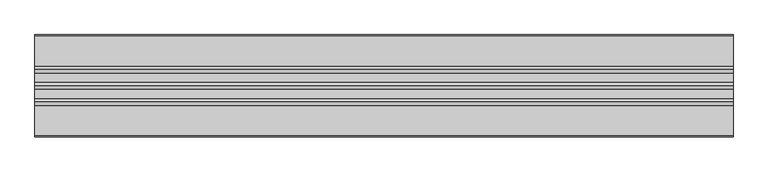
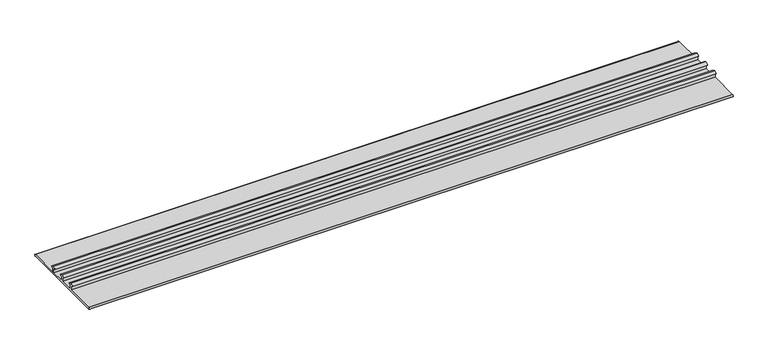
"""IFC4 building model written with IfcOpenShell, lengths in millimetres: proxy geometry, TN_ПВХ_ТПО_Гидрошпонка ТехноНИКОЛЬ : ПВХ Гидрошпонка ТехноНИКОЛЬ EC-220-3."""

import ifcopenshell
import ifcopenshell.guid

model = None  # the IFC model being written
_history = None  # IfcOwnerHistory: only IFC2X3 demands one
_inside = {}  # id of a spatial element -> (the spatial element, [elements in it])
_under = {}  # id of a project, library or spatial element -> (it, [spatial elements below it])
_declared = {}  # id of a project -> (the project, [libraries it declares])
_typed = {}  # id of a type object -> (the type object, [elements of that type])
_made_of = {}  # id of a material, layer set ... -> (it, [elements and type objects made of it])


def new_model(schema):
    """Start an empty IFC model of exactly this schema.

    Asked for "IFC4X3", IfcOpenShell would pick the latest addendum, in which some entities
    have other attributes; the version numbers below select the first issue.
    IFC2X3 requires an IfcOwnerHistory on every rooted entity: one is made here for all.
    """
    global model, _history
    if schema == "IFC4X3":
        model = ifcopenshell.file(schema_version=(4, 3, 0, 0))
    else:
        model = ifcopenshell.file(schema=schema)
    _inside.clear()
    _under.clear()
    _declared.clear()
    _typed.clear()
    _made_of.clear()
    _history = None
    if model.schema == "IFC2X3":
        org = make("IfcOrganization", Name="unknown")
        user = make(
            "IfcPersonAndOrganization",
            ThePerson=make("IfcPerson", FamilyName="unknown"),
            TheOrganization=org,
        )
        app = make(
            "IfcApplication",
            ApplicationDeveloper=org,
            Version="unknown",
            ApplicationFullName="unknown",
            ApplicationIdentifier="unknown",
        )
        _history = make(
            "IfcOwnerHistory",
            OwningUser=user,
            OwningApplication=app,
            ChangeAction="ADDED",
            CreationDate=0,
        )
    return model


def make(cls, **values):
    """One entity of the class cls with the attributes given. An attribute that is None is left unset."""
    return model.create_entity(
        cls, **{name: value for name, value in values.items() if value is not None}
    )


def rooted(cls, **values):
    """An entity with a GlobalId (a new one), such as an element, a storey or a relation."""
    return make(cls, GlobalId=ifcopenshell.guid.new(), OwnerHistory=_history, **values)


def si_unit(unit_type, name, prefix=None):
    """IfcSIUnit, for example si_unit("LENGTHUNIT", "METRE", prefix="MILLI")."""
    return make("IfcSIUnit", UnitType=unit_type, Prefix=prefix, Name=name)


def assignment(units):
    """IfcUnitAssignment: the units of a project."""
    return None if units is None else make("IfcUnitAssignment", Units=units)


def point(xyz):
    """IfcCartesianPoint."""
    return None if xyz is None else make("IfcCartesianPoint", Coordinates=xyz)


def direction(xyz):
    """IfcDirection."""
    return None if xyz is None else make("IfcDirection", DirectionRatios=xyz)


def frame(location, z_axis=None, x_axis=None):
    """IfcAxis2Placement3D, a coordinate frame: its origin and axes. An axis left out is left unset."""
    return make(
        "IfcAxis2Placement3D",
        Location=point(location),
        Axis=direction(z_axis),
        RefDirection=direction(x_axis),
    )


def frame_2d(location, x_axis=None):
    """IfcAxis2Placement2D, a coordinate frame in the plane: its origin and x axis."""
    return make(
        "IfcAxis2Placement2D", Location=point(location), RefDirection=direction(x_axis)
    )


def origin():
    """The frame at (0, 0, 0) with its axes left unset."""
    return frame((0.0, 0.0, 0.0))


def place(relative_to, where):
    """IfcLocalPlacement: puts the frame where relative to a parent placement (None: the world)."""
    return make(
        "IfcLocalPlacement", PlacementRelTo=relative_to, RelativePlacement=where
    )


def context(
    kind, dimensions, precision=None, world=None, true_north=None, identifier=None
):
    """IfcGeometricRepresentationContext, for example the 3D "Model" context."""
    return make(
        "IfcGeometricRepresentationContext",
        ContextIdentifier=identifier,
        ContextType=kind,
        CoordinateSpaceDimension=dimensions,
        Precision=precision,
        WorldCoordinateSystem=world,
        TrueNorth=true_north,
    )


def project(units=None, contexts=None):
    """IfcProject with its units and contexts."""
    return rooted(
        "IfcProject",
        Name="project",
        RepresentationContexts=contexts,
        UnitsInContext=assignment(units),
    )


def spatial(cls, under=None, at=None, **own):
    """A site, building, storey or space (cls), placed at a placement, below another one or the project."""
    s = rooted(cls, ObjectPlacement=at, **own)
    if under is not None:
        _under.setdefault(under.id(), (under, []))[1].append(s)
    return s


def polyline(points):
    """IfcPolyline through the points."""
    return make("IfcPolyline", Points=[point(p) for p in points])


def circle_curve(where, radius):
    """IfcCircle in the frame where."""
    return make("IfcCircle", Position=where, Radius=radius)


def trimmed(basis, trim1, trim2, sense, master):
    """IfcTrimmedCurve: the piece of a basis curve between two trims."""
    return make(
        "IfcTrimmedCurve",
        BasisCurve=basis,
        Trim1=trim1,
        Trim2=trim2,
        SenseAgreement=sense,
        MasterRepresentation=master,
    )


def segment(curve, same_sense, transition):
    """IfcCompositeCurveSegment."""
    return make(
        "IfcCompositeCurveSegment",
        Transition=transition,
        SameSense=same_sense,
        ParentCurve=curve,
    )


def composite_curve(segments, self_intersect=None):
    """IfcCompositeCurve: segments joined end to end."""
    return make("IfcCompositeCurve", Segments=segments, SelfIntersect=self_intersect)


def outline(outer, holes=None, kind="AREA"):
    """IfcArbitraryClosedProfileDef: a profile drawn as a closed curve; with holes, ...WithVoids."""
    if holes is None:
        return make("IfcArbitraryClosedProfileDef", ProfileType=kind, OuterCurve=outer)
    return make(
        "IfcArbitraryProfileDefWithVoids",
        ProfileType=kind,
        OuterCurve=outer,
        InnerCurves=holes,
    )


def extrude(swept, where, along, depth):
    """IfcExtrudedAreaSolid: the profile swept, set in the frame where, extruded along a direction by depth."""
    return make(
        "IfcExtrudedAreaSolid",
        SweptArea=swept,
        Position=where,
        ExtrudedDirection=direction(along),
        Depth=depth,
    )


def shape(context_of_items, identifier, shape_type, items):
    """IfcShapeRepresentation: the items that make up one representation, for example the "Body"."""
    return make(
        "IfcShapeRepresentation",
        ContextOfItems=context_of_items,
        RepresentationIdentifier=identifier,
        RepresentationType=shape_type,
        Items=items,
    )


def source(mapping_origin, context_of_items, identifier, shape_type, items):
    """IfcRepresentationMap: a shape defined once, which mapped items show again and again."""
    return make(
        "IfcRepresentationMap",
        MappingOrigin=mapping_origin,
        MappedRepresentation=shape(context_of_items, identifier, shape_type, items),
    )


def transform(
    local_origin,
    x_axis=None,
    y_axis=None,
    z_axis=None,
    scale=None,
    scale2=None,
    scale3=None,
    uniform=True,
):
    """IfcCartesianTransformationOperator3D, or its non-uniform kind. x_axis, y_axis, z_axis: its Axis1, 2, 3."""
    if uniform:
        return make(
            "IfcCartesianTransformationOperator3D",
            Axis1=direction(x_axis),
            Axis2=direction(y_axis),
            LocalOrigin=point(local_origin),
            Scale=scale,
            Axis3=direction(z_axis),
        )
    return make(
        "IfcCartesianTransformationOperator3DnonUniform",
        Axis1=direction(x_axis),
        Axis2=direction(y_axis),
        LocalOrigin=point(local_origin),
        Scale=scale,
        Axis3=direction(z_axis),
        Scale2=scale2,
        Scale3=scale3,
    )


def mapped(mapping_source, mapping_target):
    """IfcMappedItem: shows the shape of a source again, moved by a transform."""
    return make(
        "IfcMappedItem", MappingSource=mapping_source, MappingTarget=mapping_target
    )


def made_of(thing, what):
    """Note that an element or type object is made of a material, layer set ...; save() writes the relation."""
    if what is not None:
        _made_of.setdefault(what.id(), (what, []))[1].append(thing)
    return thing


def element(
    cls,
    number,
    at=None,
    inside=None,
    cuts=None,
    type_object=None,
    material=None,
    context=None,
    identifier="Body",
    shape_type=None,
    held_by="IfcProductDefinitionShape",
    body=None,
    shapes=None,
    **own,
):
    """One element of the class cls, such as IfcWall. Its Tag is "e" and its number.

    at: its placement. inside: the storey or other place that contains it. cuts: it is an
    opening in that element (IfcRelVoidsElement). A single representation is given by context,
    identifier, shape_type and body (its items); several are given by shapes. held_by: the class
    of the entity that holds the representations. save() writes the other relations.
    """
    e = rooted(cls, Tag="e%d" % number, ObjectPlacement=at, **own)
    if body is not None:
        shapes = [shape(context, identifier, shape_type, body)]
    if shapes is not None:
        e.Representation = make(held_by, Representations=shapes)
    if inside is not None:
        _inside.setdefault(inside.id(), (inside, []))[1].append(e)
    if cuts is not None:
        rooted(
            "IfcRelVoidsElement", RelatingBuildingElement=cuts, RelatedOpeningElement=e
        )
    if type_object is not None:
        _typed.setdefault(type_object.id(), (type_object, []))[1].append(e)
    return made_of(e, material)


def aggregate(whole, parts):
    """IfcRelAggregates: a whole, such as a stair, and the parts it consists of."""
    return rooted("IfcRelAggregates", RelatingObject=whole, RelatedObjects=parts)


def save(model, path):
    """Write the relations noted so far, then the file.

    IfcRelAggregates (storeys below a building ...), IfcRelContainedInSpatialStructure (elements
    in a storey), IfcRelDefinesByType, IfcRelAssociatesMaterial and IfcRelDeclares: one each for
    every whole, place, type object, material and project.
    """
    for whole, parts in _under.values():
        aggregate(whole, parts)
    for where, things in _inside.values():
        rooted(
            "IfcRelContainedInSpatialStructure",
            RelatedElements=things,
            RelatingStructure=where,
        )
    for kind, things in _typed.values():
        rooted("IfcRelDefinesByType", RelatedObjects=things, RelatingType=kind)
    for what, things in _made_of.values():
        rooted("IfcRelAssociatesMaterial", RelatedObjects=things, RelatingMaterial=what)
    for by, libraries in _declared.values():
        rooted("IfcRelDeclares", RelatingContext=by, RelatedDefinitions=libraries)
    model.write(path)


def specialty_equipment_4c86b9bd(model_context):
    return source(origin(), model_context, "Body", "SweptSolid", [
        extrude(outline(composite_curve([segment(polyline([(107.5, 0.0), (-107.5, 0.0)]), True, "CONTINUOUS"), segment(trimmed(circle_curve(frame_2d((-107.5, 2.5)), 2.5), [point((-107.5, 0.0))], [point((-107.5, 5.0))], False, "CARTESIAN"), True, "CONTINUOUS"), segment(polyline([(-107.5, 5.0), (-37.0, 5.0), (-37.0, 13.2999466), (-41.9441602, 16.7618849), (-35.0, 20.0), (-28.0558398, 16.7618849), (-33.0, 13.2999466), (-33.0, 5.0), (-2.0, 5.0), (-2.0, 13.2999466), (-6.9441602, 16.7618849), (0.0, 20.0), (6.9441602, 16.7618849), (2.0, 13.2999466), (2.0, 5.0), (33.0, 5.0), (33.0, 13.2999466), (28.0558398, 16.7618849), (35.0, 20.0), (41.9441602, 16.7618849), (37.0, 13.2999466), (37.0, 5.0), (107.5, 5.0)]), True, "CONTINUOUS"), segment(trimmed(circle_curve(frame_2d((107.5, 2.5)), 2.5), [point((107.5, 5.0))], [point((107.5, 0.0))], False, "CARTESIAN"), True, "CONTINUOUS")], self_intersect=False)), frame((0.0, 0.0, 0.0), z_axis=(1.0, 0.0, 0.0), x_axis=(0.0, 1.0, 0.0)), (0.0, 0.0, 1.0), 1500.0),
    ])


if __name__ == "__main__":
    model = new_model("IFC4")
    model_context = context("Model", 3, world=origin())
    ifc_project = project(units=[si_unit("LENGTHUNIT", "METRE", prefix="MILLI")], contexts=[model_context])
    site = spatial("IfcSite", under=ifc_project)
    building = spatial("IfcBuilding", under=site)
    placement = place(None, origin())
    specialty_equipment_shape = specialty_equipment_4c86b9bd(model_context)
    element("IfcBuildingElementProxy", 1, Name="TN_ПВХ_ТПО_Гидрошпонка ТехноНИКОЛЬ : ПВХ Гидрошпонка ТехноНИКОЛЬ EC-220-3", ObjectType="TN_ПВХ_ТПО_Гидрошпонка ТехноНИКОЛЬ : ПВХ Гидрошпонка ТехноНИКОЛЬ EC-220-3", at=placement, inside=building, context=model_context, shape_type="MappedRepresentation", body=[
        mapped(specialty_equipment_shape, transform((0.0, 0.0, 0.0), x_axis=(1.0, 0.0, 0.0), y_axis=(0.0, 1.0, 0.0), z_axis=(0.0, 0.0, 1.0))),
    ])
    save(model, "model.ifc")

# Revit data of these elements
# Type "TN_ПВХ_ТПО_Гидрошпонка ТехноНИКОЛЬ : ПВХ Гидрошпонка ТехноНИКОЛЬ EC-220-3"
#   Description = "Наружная гидрошпонка применяется для герметизации рабочих швов бетонирования и для разбивки на секции (карты) гидроизоляционных систем на основе ПВХ мембран LOGICBASE V-SL"
#   Type Comments = "п.м."
#   Manufacturer = "ТехноНИКОЛЬ"
#   URL = "https://shop.tn.ru/pvh-gidroshponka-ec-220-3-20-m-rul"
#   ADSK_Примечание = ""
#   ADSK_Обозначение [instance default] = "ТехноНИКОЛЬ"
#   ADSK_Наименование = "ПВХ Гидрошпонка ТехноНИКОЛЬ EC-220-3, 20м/рул"
#   ADSK_Масса_Текст = ""
#   ADSK_Марка = ""
#   ADSK_Код изделия = "499876"
#   ADSK_Завод-изготовитель [instance default] = "ТехноНИКОЛЬ"
#   ADSK_Единица измерения [instance default] = "п.м."
#   ADSK_Группирование = "Гидрошпонки"
#   ADSK_URL страницы изделия = "https://shop.tn.ru/pvh-gidroshponka-ec-220-3-20-m-rul"
#   ADSK_URL документации изделия = "https://nav.tn.ru/upload/iblock/67f/Katalog-i-rekomendatsii-po-primeneniyu_Gidroshponki-TEKHNONIKOL.PDF"
#   built-in parameter 1001306 [instance default] = 3.28084 (stored number, unit not read)
#   ADSK_Размер_Длина [instance default] = 1000 mm
#   ADSK_Количество [instance default] = 1
#   ПВХ_ТПО Гидрошпонка ТехноНИКОЛЬ EC-320-4 = no
#   ПВХ Гидрошпонка ТехноНИКОЛЬ IM-260/50 = no
#   ПВХ Гидрошпонка ТехноНИКОЛЬ IM-240/20 = no
#   ПВХ Гидрошпонка ТехноНИКОЛЬ IC-240-6 = no
#   ПВХ Гидрошпонка ТехноНИКОЛЬ IC-125-2SP = no
#   ПВХ Гидрошпонка ТехноНИКОЛЬ EM-260/50 = no
#   ПВХ Гидрошпонка ТехноНИКОЛЬ EM-260/20 = no
#   ПВХ Гидрошпонка ТехноНИКОЛЬ EC-320-4 = no
#   ПВХ Гидрошпонка ТехноНИКОЛЬ EC-220-3 = no
#   ПВХ_ТПО Гидрошпонка ТехноНИКОЛЬ EC-220-3 = yes
#   ПВХ Гидрошпонка ТехноНИКОЛЬ IC-240-2 = no
#   Материал = TN_ПВХ_Черный
#   Default Elevation = 0
# Element 1 (IfcBuildingElementProxy, "TN_ПВХ_ТПО_Гидрошпонка ТехноНИКОЛЬ : ПВХ Гидрошпонка ТехноНИКОЛЬ EC-220-3")
#   built-in parameter 1001306 = 4.92126 (stored number, unit not read)
#   ADSK_Размер_Длина = 1500 mm
#   ADSK_Количество = 1.5
#   Materials on its faces: "TN_ПВХ_Черный"
# Materials
#   "TN_ПВХ_Черный": class "Типовые", colour RGB 48 48 48, transparency 0, Cost = 0
